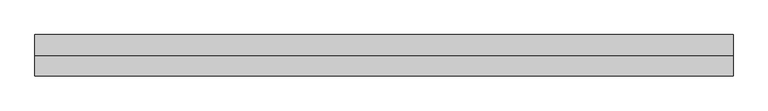
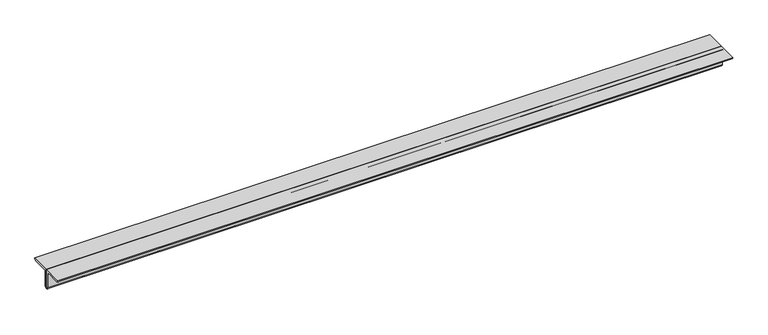
"""IFC4 building model written with IfcOpenShell, lengths in millimetres: member geometry, 0123_Steel Framing_2Ls-KSD3502 : H_SB_AR_S03_2Ls-130x130x12_HBR1."""

from ifc_helpers import new_model, si_unit, point, frame, frame_2d, origin, place, context, project, spatial, polyline, circle_curve, trimmed, segment, composite_curve, outline, extrude, source, transform, mapped, element, save


def member_e19a7e3f(model_context):
    return source(origin(), model_context, "Body", "SweptSolid", [
        extrude(outline(composite_curve([segment(polyline([(0.0, 36.4), (130.0, 36.4)]), True, "CONTINUOUS"), segment(trimmed(circle_curve(frame_2d((118.0, 36.4)), 12.0), [point((130.0, 36.4))], [point((118.0, 24.4))], False, "CARTESIAN"), True, "CONTINUOUS"), segment(polyline([(118.0, 24.4), (24.0, 24.4)]), True, "CONTINUOUS"), segment(trimmed(circle_curve(frame_2d((24.0, 12.4)), 12.0), [point((24.0, 24.4))], [point((12.0, 12.4))], True, "CARTESIAN"), True, "CONTINUOUS"), segment(polyline([(12.0, 12.4), (12.0, -81.6)]), True, "CONTINUOUS"), segment(trimmed(circle_curve(frame_2d((0.0, -81.6)), 12.0), [point((12.0, -81.6))], [point((0.0, -93.6))], False, "CARTESIAN"), True, "CONTINUOUS"), segment(polyline([(0.0, -93.6), (0.0, 36.4)]), True, "CONTINUOUS")], self_intersect=False)), frame((-2158.4448527, 0.0, 0.0), z_axis=(1.0, 0.0, 0.0), x_axis=(0.0, 1.0, 0.0)), (0.0, 0.0, 1.0), 4391.0649986),
        extrude(outline(composite_curve([segment(polyline([(0.0, 36.4), (0.0, -93.6)]), True, "CONTINUOUS"), segment(trimmed(circle_curve(frame_2d((0.0, -81.6)), 12.0), [point((0.0, -93.6))], [point((-12.0, -81.6))], False, "CARTESIAN"), True, "CONTINUOUS"), segment(polyline([(-12.0, -81.6), (-12.0, 12.4)]), True, "CONTINUOUS"), segment(trimmed(circle_curve(frame_2d((-24.0, 12.4)), 12.0), [point((-12.0, 12.4))], [point((-24.0, 24.4))], True, "CARTESIAN"), True, "CONTINUOUS"), segment(polyline([(-24.0, 24.4), (-118.0, 24.4)]), True, "CONTINUOUS"), segment(trimmed(circle_curve(frame_2d((-118.0, 36.4)), 12.0), [point((-118.0, 24.4))], [point((-130.0, 36.4))], False, "CARTESIAN"), True, "CONTINUOUS"), segment(polyline([(-130.0, 36.4), (0.0, 36.4)]), True, "CONTINUOUS")], self_intersect=False)), frame((-2158.4448527, 0.0, 0.0), z_axis=(1.0, 0.0, 0.0), x_axis=(0.0, 1.0, 0.0)), (0.0, 0.0, 1.0), 4391.0649986),
    ])


if __name__ == "__main__":
    model = new_model("IFC4")
    model_context = context("Model", 3, world=origin())
    ifc_project = project(units=[si_unit("LENGTHUNIT", "METRE", prefix="MILLI")], contexts=[model_context])
    site = spatial("IfcSite", under=ifc_project)
    building = spatial("IfcBuilding", under=site)
    placement = place(None, origin())
    member_shape = member_e19a7e3f(model_context)
    element("IfcMember", 1, ObjectType="0123_Steel Framing_2Ls-KSD3502 : H_SB_AR_S03_2Ls-130x130x12_HBR1", at=placement, inside=building, context=model_context, shape_type="MappedRepresentation", body=[
        mapped(member_shape, transform((0.0, 0.0, 0.0), x_axis=(1.0, 0.0, 0.0), y_axis=(0.0, 1.0, 0.0), z_axis=(0.0, 0.0, 1.0))),
    ])
    save(model, "model.ifc")

# Revit data of these elements
# Type "0123_Steel Framing_2Ls-KSD3502 : H_SB_AR_S03_2Ls-130x130x12_HBR1"
#   Assembly Code = "B10"
#   Legs = "SLBB"
#   W = 8.97
#   Perimeter = 1.04 m²/m
#   Nominal Weight = 46.80 kgf/m
#   Length [instance default] = 1000 mm
#   Space = 0 mm
#   b = 130 mm
#   d = 130 mm
#   t = 12 mm
#   y = 36.4 mm
#   A = 0.005952 m²
#   Structural Material [instance default] = Steel ASTM A36
# Element 1 (IfcMember, "0123_Steel Framing_2Ls-KSD3502 : H_SB_AR_S03_2Ls-130x130x12_HBR1")
#   Structural Material = Steel, 45-345
#   Materials on its faces: "Steel, 45-345"
# Materials
#   "Steel ASTM A36": class "Metal", colour RGB 199 199 199, transparency 0, Description = "Structural steel, ASTM A36 Grade B, mill finish", Cost = 0
#   "Steel, 45-345": class "Metal", colour RGB 189 187 185, transparency 0, Description = "Steel 345 MPa", Cost = 0
